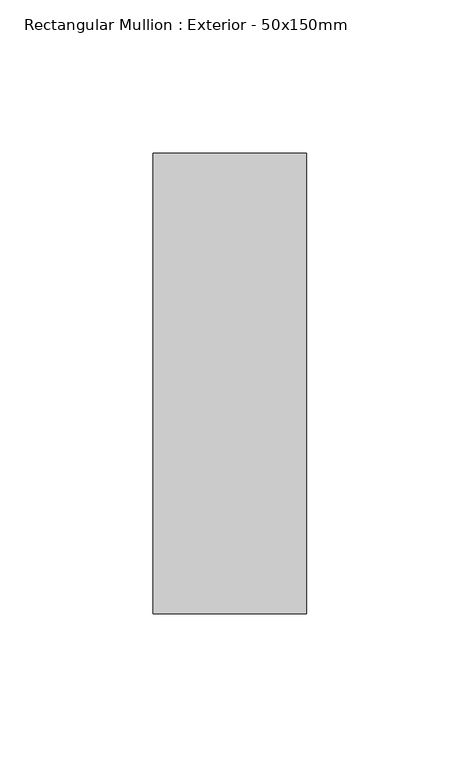
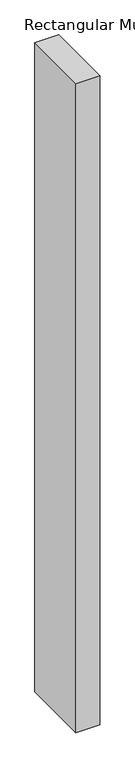
"""IFC4 building model written with IfcOpenShell, lengths in millimetres: member geometry, Rectangular Mullion : Exterior - 50x150mm."""

from ifc_helpers import new_model, si_unit, frame, origin, place, context, project, spatial, polyline, outline, extrude, source, transform, mapped, element, save


def rectangular_mullion_exterior_50x150mm_99e7c456(model_context):
    return source(origin(), model_context, "Body", "SweptSolid", [
        extrude(outline(polyline([(25.0, 0.0), (25.0, -150.0), (-25.0, -150.0), (-25.0, 0.0), (25.0, 0.0)])), frame((0.0, 0.0, -1449.9999999), z_axis=(0.0, 0.0, 1.0), x_axis=(1.0, 0.0, 0.0)), (0.0, 0.0, 1.0), 1449.9999999),
    ])


if __name__ == "__main__":
    model = new_model("IFC4")
    model_context = context("Model", 3, world=origin())
    ifc_project = project(units=[si_unit("LENGTHUNIT", "METRE", prefix="MILLI")], contexts=[model_context])
    site = spatial("IfcSite", under=ifc_project)
    building = spatial("IfcBuilding", under=site)
    placement = place(None, origin())
    rectangular_mullion_exterior_50x150mm_shape = rectangular_mullion_exterior_50x150mm_99e7c456(model_context)
    element("IfcMember", 1, ObjectType="Rectangular Mullion : Exterior - 50x150mm", at=placement, inside=building, context=model_context, shape_type="MappedRepresentation", body=[
        mapped(rectangular_mullion_exterior_50x150mm_shape, transform((0.0, 0.0, 0.0), x_axis=(1.0, 0.0, 0.0), y_axis=(0.0, 1.0, 0.0), z_axis=(0.0, 0.0, 1.0))),
    ])
    save(model, "model.ifc")

# Revit data of these elements
# Type "Rectangular Mullion : Exterior - 50x150mm"
#   built-in parameter 1007351 = -0.246063 (stored number, unit not read)
#   built-in parameter 1007304 = 0.492126 (stored number, unit not read)
#   built-in parameter 1007301 = 0.082021 (stored number, unit not read)
#   built-in parameter 1007300 = 0.082021 (stored number, unit not read)
# Element 1 (IfcMember, "Rectangular Mullion : Exterior - 50x150mm")
#   Materials on its faces: "Default Frame/Mullion (Interior/Exterior)"
# Materials
#   "Default Frame/Mullion (Interior/Exterior)": class "Generic", colour RGB 205 205 205, transparency 0, Description = "Udefineret karm/ramme materiale", Cost = 0
